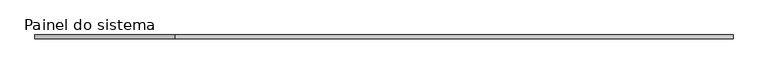
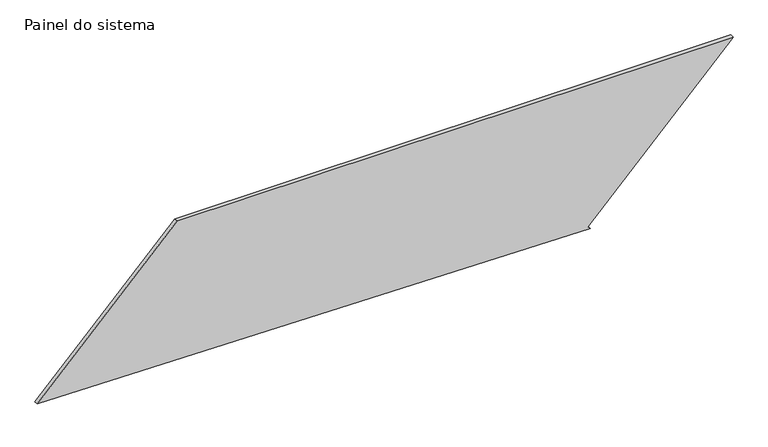
"""IFC4 building model written with IfcOpenShell, lengths in millimetres: plate geometry, Painel do sistema : Envidraçado."""

from ifc_helpers import new_model, si_unit, frame, origin, place, context, project, spatial, polyline, outline, extrude, source, transform, mapped, element, save


def painel_do_sistema_bace2d31(model_context):
    return source(origin(), model_context, "Body", "SweptSolid", [
        extrude(outline(polyline([(0.0, 1310.041954), (17.3932625, 1292.0843813), (975.1849867, 2219.7778498), (975.1849867, -1326.9555993), (53.3958487, -2219.7778498), (0.0, 1310.041954)])), frame((0.0, 24.5, 0.0), z_axis=(0.0, 1.0, 0.0), x_axis=(0.0, 0.0, 1.0)), (0.0, 0.0, 1.0), 25.0),
    ])


if __name__ == "__main__":
    model = new_model("IFC4")
    model_context = context("Model", 3, world=origin())
    ifc_project = project(units=[si_unit("LENGTHUNIT", "METRE", prefix="MILLI")], contexts=[model_context])
    site = spatial("IfcSite", under=ifc_project)
    building = spatial("IfcBuilding", under=site)
    placement = place(None, origin())
    painel_do_sistema_shape = painel_do_sistema_bace2d31(model_context)
    element("IfcPlate", 1, ObjectType="Painel do sistema : Envidraçado", at=placement, inside=building, context=model_context, shape_type="MappedRepresentation", body=[
        mapped(painel_do_sistema_shape, transform((0.0, 0.0, 0.0), x_axis=(1.0, 0.0, 0.0), y_axis=(0.0, 1.0, 0.0), z_axis=(0.0, 0.0, 1.0))),
    ])
    save(model, "model.ifc")

# Revit data of these elements
# Type "Painel do sistema : Envidraçado"
#   Construction Type Id = "GSP4R"
#   Analytic Construction = "Vidraça única Pilkington 1/8 pol"
#   Visual Light Transmittance = 0.9
#   Solar Heat Gain Coefficient = 0.86
#   Heat Transfer Coefficient (U) = 6.7069 W/(m²·K)
# Element 1 (IfcPlate, "Painel do sistema : Envidraçado")
#   Materials on its faces: "Vidro"
# Materials
#   "Vidro": class "Vidro", colour RGB 0 128 192, transparency 0.9, Description = "Vidro de sílica", Cost = 0
